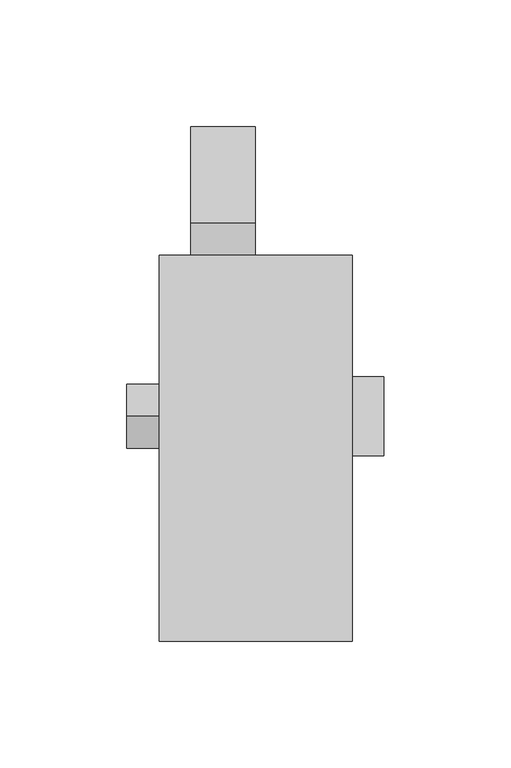
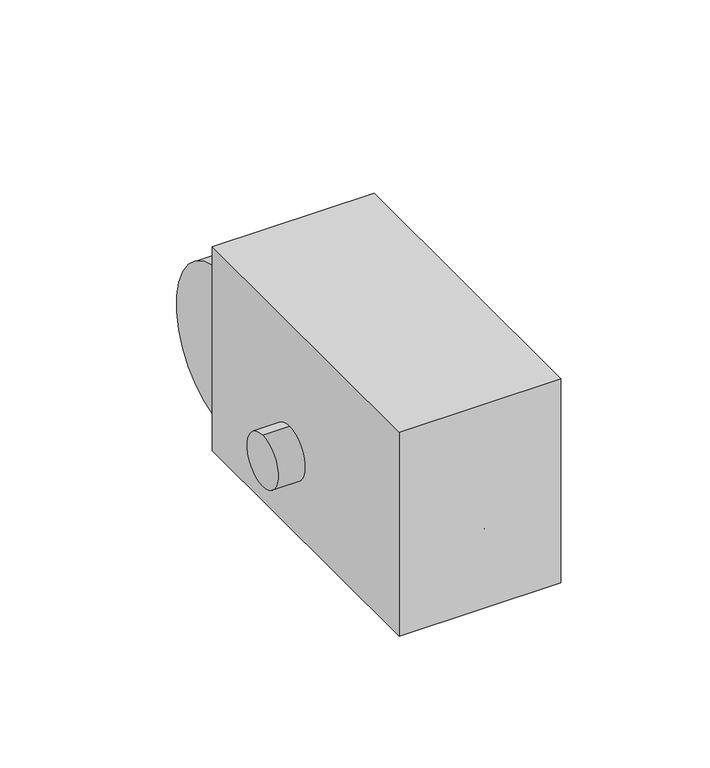
"""IFC4 building model written with IfcOpenShell, lengths in millimetres: proxy geometry, M0765 - Regulator, Vacuum : M0765 - Regulator, Vacuum."""

import ifcopenshell
import ifcopenshell.guid

model = None  # the IFC model being written
_history = None  # IfcOwnerHistory: only IFC2X3 demands one
_inside = {}  # id of a spatial element -> (the spatial element, [elements in it])
_under = {}  # id of a project, library or spatial element -> (it, [spatial elements below it])
_declared = {}  # id of a project -> (the project, [libraries it declares])
_typed = {}  # id of a type object -> (the type object, [elements of that type])
_made_of = {}  # id of a material, layer set ... -> (it, [elements and type objects made of it])


def new_model(schema):
    """Start an empty IFC model of exactly this schema.

    Asked for "IFC4X3", IfcOpenShell would pick the latest addendum, in which some entities
    have other attributes; the version numbers below select the first issue.
    IFC2X3 requires an IfcOwnerHistory on every rooted entity: one is made here for all.
    """
    global model, _history
    if schema == "IFC4X3":
        model = ifcopenshell.file(schema_version=(4, 3, 0, 0))
    else:
        model = ifcopenshell.file(schema=schema)
    _inside.clear()
    _under.clear()
    _declared.clear()
    _typed.clear()
    _made_of.clear()
    _history = None
    if model.schema == "IFC2X3":
        org = make("IfcOrganization", Name="unknown")
        user = make(
            "IfcPersonAndOrganization",
            ThePerson=make("IfcPerson", FamilyName="unknown"),
            TheOrganization=org,
        )
        app = make(
            "IfcApplication",
            ApplicationDeveloper=org,
            Version="unknown",
            ApplicationFullName="unknown",
            ApplicationIdentifier="unknown",
        )
        _history = make(
            "IfcOwnerHistory",
            OwningUser=user,
            OwningApplication=app,
            ChangeAction="ADDED",
            CreationDate=0,
        )
    return model


def make(cls, **values):
    """One entity of the class cls with the attributes given. An attribute that is None is left unset."""
    return model.create_entity(
        cls, **{name: value for name, value in values.items() if value is not None}
    )


def rooted(cls, **values):
    """An entity with a GlobalId (a new one), such as an element, a storey or a relation."""
    return make(cls, GlobalId=ifcopenshell.guid.new(), OwnerHistory=_history, **values)


def si_unit(unit_type, name, prefix=None):
    """IfcSIUnit, for example si_unit("LENGTHUNIT", "METRE", prefix="MILLI")."""
    return make("IfcSIUnit", UnitType=unit_type, Prefix=prefix, Name=name)


def assignment(units):
    """IfcUnitAssignment: the units of a project."""
    return None if units is None else make("IfcUnitAssignment", Units=units)


def point(xyz):
    """IfcCartesianPoint."""
    return None if xyz is None else make("IfcCartesianPoint", Coordinates=xyz)


def direction(xyz):
    """IfcDirection."""
    return None if xyz is None else make("IfcDirection", DirectionRatios=xyz)


def frame(location, z_axis=None, x_axis=None):
    """IfcAxis2Placement3D, a coordinate frame: its origin and axes. An axis left out is left unset."""
    return make(
        "IfcAxis2Placement3D",
        Location=point(location),
        Axis=direction(z_axis),
        RefDirection=direction(x_axis),
    )


def frame_2d(location, x_axis=None):
    """IfcAxis2Placement2D, a coordinate frame in the plane: its origin and x axis."""
    return make(
        "IfcAxis2Placement2D", Location=point(location), RefDirection=direction(x_axis)
    )


def origin():
    """The frame at (0, 0, 0) with its axes left unset."""
    return frame((0.0, 0.0, 0.0))


def origin_with_axes():
    """The frame at (0, 0, 0) with the z axis (0, 0, 1) and the x axis (1, 0, 0) written out."""
    return frame((0.0, 0.0, 0.0), z_axis=(0.0, 0.0, 1.0), x_axis=(1.0, 0.0, 0.0))


def place(relative_to, where):
    """IfcLocalPlacement: puts the frame where relative to a parent placement (None: the world)."""
    return make(
        "IfcLocalPlacement", PlacementRelTo=relative_to, RelativePlacement=where
    )


def context(
    kind, dimensions, precision=None, world=None, true_north=None, identifier=None
):
    """IfcGeometricRepresentationContext, for example the 3D "Model" context."""
    return make(
        "IfcGeometricRepresentationContext",
        ContextIdentifier=identifier,
        ContextType=kind,
        CoordinateSpaceDimension=dimensions,
        Precision=precision,
        WorldCoordinateSystem=world,
        TrueNorth=true_north,
    )


def project(units=None, contexts=None):
    """IfcProject with its units and contexts."""
    return rooted(
        "IfcProject",
        Name="project",
        RepresentationContexts=contexts,
        UnitsInContext=assignment(units),
    )


def spatial(cls, under=None, at=None, **own):
    """A site, building, storey or space (cls), placed at a placement, below another one or the project."""
    s = rooted(cls, ObjectPlacement=at, **own)
    if under is not None:
        _under.setdefault(under.id(), (under, []))[1].append(s)
    return s


def polyline(points):
    """IfcPolyline through the points."""
    return make("IfcPolyline", Points=[point(p) for p in points])


def circle_curve(where, radius):
    """IfcCircle in the frame where."""
    return make("IfcCircle", Position=where, Radius=radius)


def trimmed(basis, trim1, trim2, sense, master):
    """IfcTrimmedCurve: the piece of a basis curve between two trims."""
    return make(
        "IfcTrimmedCurve",
        BasisCurve=basis,
        Trim1=trim1,
        Trim2=trim2,
        SenseAgreement=sense,
        MasterRepresentation=master,
    )


def segment(curve, same_sense, transition):
    """IfcCompositeCurveSegment."""
    return make(
        "IfcCompositeCurveSegment",
        Transition=transition,
        SameSense=same_sense,
        ParentCurve=curve,
    )


def composite_curve(segments, self_intersect=None):
    """IfcCompositeCurve: segments joined end to end."""
    return make("IfcCompositeCurve", Segments=segments, SelfIntersect=self_intersect)


def outline(outer, holes=None, kind="AREA"):
    """IfcArbitraryClosedProfileDef: a profile drawn as a closed curve; with holes, ...WithVoids."""
    if holes is None:
        return make("IfcArbitraryClosedProfileDef", ProfileType=kind, OuterCurve=outer)
    return make(
        "IfcArbitraryProfileDefWithVoids",
        ProfileType=kind,
        OuterCurve=outer,
        InnerCurves=holes,
    )


def extrude(swept, where, along, depth):
    """IfcExtrudedAreaSolid: the profile swept, set in the frame where, extruded along a direction by depth."""
    return make(
        "IfcExtrudedAreaSolid",
        SweptArea=swept,
        Position=where,
        ExtrudedDirection=direction(along),
        Depth=depth,
    )


def shape(context_of_items, identifier, shape_type, items):
    """IfcShapeRepresentation: the items that make up one representation, for example the "Body"."""
    return make(
        "IfcShapeRepresentation",
        ContextOfItems=context_of_items,
        RepresentationIdentifier=identifier,
        RepresentationType=shape_type,
        Items=items,
    )


def source(mapping_origin, context_of_items, identifier, shape_type, items):
    """IfcRepresentationMap: a shape defined once, which mapped items show again and again."""
    return make(
        "IfcRepresentationMap",
        MappingOrigin=mapping_origin,
        MappedRepresentation=shape(context_of_items, identifier, shape_type, items),
    )


def transform(
    local_origin,
    x_axis=None,
    y_axis=None,
    z_axis=None,
    scale=None,
    scale2=None,
    scale3=None,
    uniform=True,
):
    """IfcCartesianTransformationOperator3D, or its non-uniform kind. x_axis, y_axis, z_axis: its Axis1, 2, 3."""
    if uniform:
        return make(
            "IfcCartesianTransformationOperator3D",
            Axis1=direction(x_axis),
            Axis2=direction(y_axis),
            LocalOrigin=point(local_origin),
            Scale=scale,
            Axis3=direction(z_axis),
        )
    return make(
        "IfcCartesianTransformationOperator3DnonUniform",
        Axis1=direction(x_axis),
        Axis2=direction(y_axis),
        LocalOrigin=point(local_origin),
        Scale=scale,
        Axis3=direction(z_axis),
        Scale2=scale2,
        Scale3=scale3,
    )


def mapped(mapping_source, mapping_target):
    """IfcMappedItem: shows the shape of a source again, moved by a transform."""
    return make(
        "IfcMappedItem", MappingSource=mapping_source, MappingTarget=mapping_target
    )


def made_of(thing, what):
    """Note that an element or type object is made of a material, layer set ...; save() writes the relation."""
    if what is not None:
        _made_of.setdefault(what.id(), (what, []))[1].append(thing)
    return thing


def element(
    cls,
    number,
    at=None,
    inside=None,
    cuts=None,
    type_object=None,
    material=None,
    context=None,
    identifier="Body",
    shape_type=None,
    held_by="IfcProductDefinitionShape",
    body=None,
    shapes=None,
    **own,
):
    """One element of the class cls, such as IfcWall. Its Tag is "e" and its number.

    at: its placement. inside: the storey or other place that contains it. cuts: it is an
    opening in that element (IfcRelVoidsElement). A single representation is given by context,
    identifier, shape_type and body (its items); several are given by shapes. held_by: the class
    of the entity that holds the representations. save() writes the other relations.
    """
    e = rooted(cls, Tag="e%d" % number, ObjectPlacement=at, **own)
    if body is not None:
        shapes = [shape(context, identifier, shape_type, body)]
    if shapes is not None:
        e.Representation = make(held_by, Representations=shapes)
    if inside is not None:
        _inside.setdefault(inside.id(), (inside, []))[1].append(e)
    if cuts is not None:
        rooted(
            "IfcRelVoidsElement", RelatingBuildingElement=cuts, RelatedOpeningElement=e
        )
    if type_object is not None:
        _typed.setdefault(type_object.id(), (type_object, []))[1].append(e)
    return made_of(e, material)


def aggregate(whole, parts):
    """IfcRelAggregates: a whole, such as a stair, and the parts it consists of."""
    return rooted("IfcRelAggregates", RelatingObject=whole, RelatedObjects=parts)


def save(model, path):
    """Write the relations noted so far, then the file.

    IfcRelAggregates (storeys below a building ...), IfcRelContainedInSpatialStructure (elements
    in a storey), IfcRelDefinesByType, IfcRelAssociatesMaterial and IfcRelDeclares: one each for
    every whole, place, type object, material and project.
    """
    for whole, parts in _under.values():
        aggregate(whole, parts)
    for where, things in _inside.values():
        rooted(
            "IfcRelContainedInSpatialStructure",
            RelatedElements=things,
            RelatingStructure=where,
        )
    for kind, things in _typed.values():
        rooted("IfcRelDefinesByType", RelatedObjects=things, RelatingType=kind)
    for what, things in _made_of.values():
        rooted("IfcRelAssociatesMaterial", RelatedObjects=things, RelatingMaterial=what)
    for by, libraries in _declared.values():
        rooted("IfcRelDeclares", RelatingContext=by, RelatedDefinitions=libraries)
    model.write(path)


def plane_surface(at):
    """IfcPlane: the flat surface through the origin of the frame at, square to its z axis."""
    return make("IfcPlane", Position=at)


def cylinder_surface(at, radius):
    """IfcCylindricalSurface: all points at the distance radius from the z axis of the frame at."""
    return make("IfcCylindricalSurface", Position=at, Radius=radius)


def revolved_surface(curve, axis_point, axis_direction):
    """IfcSurfaceOfRevolution: the curve turned about the line through axis_point along axis_direction."""
    return make(
        "IfcSurfaceOfRevolution",
        SweptCurve=make("IfcArbitraryOpenProfileDef", ProfileType="CURVE", Curve=curve),
        AxisPosition=make("IfcAxis1Placement", Location=point(axis_point), Axis=direction(axis_direction)),
    )


def advanced_brep(points, edges, surfaces, faces):
    """IfcAdvancedBrep: a solid bounded by faces that lie on surfaces and meet in shared edges.

    An edge is (start, end): straight between two places in points (the first is 0);
    or (start, end, curve); or (start, end, curve, False) where it runs against its curve.
    A face is (place in surfaces, loops), or (place, loops, False) where it looks against
    its surface's normal. A loop lists edges by number (the first is 1), with a minus sign
    where the edge is run from its end to its start. The first loop is the outer one.
    """
    corners = [point(p) for p in points]
    vertices = [make("IfcVertexPoint", VertexGeometry=c) for c in corners]
    made = []
    for start, end, *more in edges:
        made.append(
            make(
                "IfcEdgeCurve",
                EdgeStart=vertices[start],
                EdgeEnd=vertices[end],
                EdgeGeometry=more[0] if more else make("IfcPolyline", Points=[corners[start], corners[end]]),
                SameSense=more[1] if len(more) > 1 else True,
            )
        )
    hull = []
    for where, loops, *sense in faces:
        bounds = []
        for j, loop in enumerate(loops):
            ring = [make("IfcOrientedEdge", EdgeElement=made[abs(k) - 1], Orientation=k > 0) for k in loop]
            bounds.append(
                make(
                    "IfcFaceOuterBound" if j == 0 else "IfcFaceBound",
                    Bound=make("IfcEdgeLoop", EdgeList=ring),
                    Orientation=True,
                )
            )
        hull.append(make("IfcAdvancedFace", Bounds=bounds, FaceSurface=surfaces[where], SameSense=sense[0] if sense else True))
    return make("IfcAdvancedBrep", Outer=make("IfcClosedShell", CfsFaces=hull))


def specialty_equipment_494a7e5c(model_context):
    return source(origin(), model_context, "Body", "SolidModel", [
        extrude(outline(polyline([(38.1, 152.4), (38.1, 0.0), (-38.1, 0.0), (-38.1, 152.4), (38.1, 152.4)])), origin_with_axes(), (0.0, 0.0, 1.0), 101.6),
        advanced_brep(
        [(-0.2368425, 76.2, 53.3223414), (-0.2368425, 76.2, 22.8776586), (-0.2368425, 76.2, 38.1), (-0.2368425, 31.8738169, 53.3223414), (-0.2368425, 31.8738169, 22.8776586), (-0.2368425, 31.8738169, 43.8248613), (-0.2368425, 31.8738169, 32.3751387), (-0.2368425, 9.172523, 43.8248613), (-0.2368425, 9.172523, 32.3751387), (-0.2368425, 9.172523, 40.8134652), (-0.2368425, 9.172523, 35.3865348), (-0.2368425, 0.0, 40.8134652), (-0.2368425, 0.0, 35.3865348), (-0.2368425, 0.0, 38.1)],
        [
            (0, 1, circle_curve(frame((-0.2368425, 76.2, 38.1), z_axis=(0.0, 1.0, 0.0), x_axis=(0.0, 0.0, -1.0)), 15.2223414)),
            (1, 2),
            (2, 0),
            (1, 0, circle_curve(frame((-0.2368425, 76.2, 38.1), z_axis=(0.0, 1.0, 0.0), x_axis=(0.0, 0.0, -1.0)), 15.2223414)),
            (3, 4, circle_curve(frame((-0.2368425, 31.8738169, 38.1), z_axis=(0.0, 1.0, 0.0), x_axis=(0.0, 0.0, -1.0)), 15.2223414)),
            (4, 1),
            (0, 3),
            (4, 3, circle_curve(frame((-0.2368425, 31.8738169, 38.1), z_axis=(0.0, 1.0, 0.0), x_axis=(0.0, 0.0, -1.0)), 15.2223414)),
            (5, 6, circle_curve(frame((-0.2368425, 31.8738169, 38.1), z_axis=(0.0, 1.0, 0.0), x_axis=(0.0, 0.0, -1.0)), 5.7248613)),
            (6, 4),
            (3, 5),
            (6, 5, circle_curve(frame((-0.2368425, 31.8738169, 38.1), z_axis=(0.0, 1.0, 0.0), x_axis=(0.0, 0.0, -1.0)), 5.7248613)),
            (7, 8, circle_curve(frame((-0.2368425, 9.172523, 38.1), z_axis=(0.0, 1.0, 0.0), x_axis=(0.0, 0.0, -1.0)), 5.7248613)),
            (8, 6),
            (5, 7),
            (8, 7, circle_curve(frame((-0.2368425, 9.172523, 38.1), z_axis=(0.0, 1.0, 0.0), x_axis=(0.0, 0.0, -1.0)), 5.7248613)),
            (9, 10, circle_curve(frame((-0.2368425, 9.172523, 38.1), z_axis=(0.0, 1.0, 0.0), x_axis=(0.0, 0.0, -1.0)), 2.7134652)),
            (10, 8),
            (7, 9),
            (10, 9, circle_curve(frame((-0.2368425, 9.172523, 38.1), z_axis=(0.0, 1.0, 0.0), x_axis=(0.0, 0.0, -1.0)), 2.7134652)),
            (11, 12, circle_curve(frame((-0.2368425, 0.0, 38.1), z_axis=(0.0, 1.0, 0.0), x_axis=(0.0, 0.0, -1.0)), 2.7134652)),
            (12, 10),
            (9, 11),
            (12, 11, circle_curve(frame((-0.2368425, 0.0, 38.1), z_axis=(0.0, 1.0, 0.0), x_axis=(0.0, 0.0, -1.0)), 2.7134652)),
            (13, 12),
            (11, 13),
        ],
        [
            plane_surface(frame((-0.2368425, 76.2, 38.1), z_axis=(0.0, 1.0, 0.0), x_axis=(0.0, 0.0, -1.0))),
            cylinder_surface(frame((-0.2368425, 1297.7300755, 38.1), z_axis=(0.0, -1.0, 0.0), x_axis=(0.0, 0.0, -1.0)), 15.2223414),
            plane_surface(frame((-0.2368425, 31.8738169, 38.1), z_axis=(0.0, -1.0, 0.0), x_axis=(0.0, 0.0, -1.0))),
            cylinder_surface(frame((-0.2368425, 1297.7300755, 38.1), z_axis=(0.0, -1.0, 0.0), x_axis=(0.0, 0.0, -1.0)), 5.7248613),
            plane_surface(frame((-0.2368425, 9.172523, 38.1), z_axis=(0.0, -1.0, 0.0), x_axis=(0.0, 0.0, -1.0))),
            cylinder_surface(frame((-0.2368425, 1297.7300755, 38.1), z_axis=(0.0, -1.0, 0.0), x_axis=(0.0, 0.0, -1.0)), 2.7134652),
            plane_surface(frame((-0.2368425, 0.0, 38.1), z_axis=(0.0, -1.0, 0.0), x_axis=(0.0, 0.0, -1.0))),
        ],
        [
            (0, [[1, 2, 3]]),
            (0, [[4, -3, -2]]),
            (1, [[5, 6, -1, 7]]),
            (1, [[8, -7, -4, -6]]),
            (2, [[9, 10, -5, 11]]),
            (2, [[12, -11, -8, -10]]),
            (3, [[13, 14, -9, 15]]),
            (3, [[16, -15, -12, -14]]),
            (4, [[17, 18, -13, 19]]),
            (4, [[20, -19, -16, -18]]),
            (5, [[21, 22, -17, 23]]),
            (5, [[24, -23, -20, -22]]),
            (6, [[25, -21, 26]]),
            (6, [[-26, -24, -25]]),
        ],
    ),
        advanced_brep(
        [(50.5631575, 104.5493597, 38.1), (50.5631575, 73.2506403, 38.1), (22.2137978, 73.2506403, 38.1), (22.2137978, 104.5493597, 38.1), (50.5631575, 88.9, 38.1), (-0.2368425, 127.0, 38.1), (-0.2368425, 50.8, 38.1), (-0.2368425, 88.9, 38.1)],
        [
            (0, 1, circle_curve(frame((50.5631575, 88.9, 38.1), z_axis=(-1.0, 0.0, 0.0), x_axis=(0.0, -1.0, 0.0)), 15.6493597)),
            (1, 2),
            (2, 3, circle_curve(frame((22.2137978, 88.9, 38.1), z_axis=(1.0, 0.0, 0.0), x_axis=(0.0, -1.0, 0.0)), 15.6493597)),
            (3, 0),
            (1, 0, circle_curve(frame((50.5631575, 88.9, 38.1), z_axis=(-1.0, 0.0, 0.0), x_axis=(0.0, -1.0, 0.0)), 15.6493597)),
            (3, 2, circle_curve(frame((22.2137978, 88.9, 38.1), z_axis=(1.0, 0.0, 0.0), x_axis=(0.0, -1.0, 0.0)), 15.6493597)),
            (4, 1),
            (0, 4),
            (5, 6, circle_curve(frame((-0.2368425, 88.9, 38.1), z_axis=(-1.0, 0.0, 0.0), x_axis=(0.0, -1.0, 0.0)), 38.1)),
            (6, 7),
            (7, 5),
            (6, 5, circle_curve(frame((-0.2368425, 88.9, 38.1), z_axis=(-1.0, 0.0, 0.0), x_axis=(0.0, -1.0, 0.0)), 38.1)),
            (2, 6),
            (5, 3),
        ],
        [
            cylinder_surface(frame((-51.0368425, 88.9, 38.1), z_axis=(1.0, 0.0, 0.0), x_axis=(0.0, -1.0, 0.0)), 15.6493597),
            plane_surface(frame((50.5631575, 88.9, 38.1), z_axis=(1.0, 0.0, 0.0), x_axis=(0.0, -1.0, 0.0))),
            plane_surface(frame((-0.2368425, 88.9, 38.1), z_axis=(-1.0, 0.0, 0.0), x_axis=(0.0, -1.0, 0.0))),
            revolved_surface(polyline([(-0.2368425, 50.8, 38.1), (22.2137978, 73.2506403, 38.1)]), (-51.0368425, 88.9, 38.1), (1.0, 0.0, 0.0)),
        ],
        [
            (0, [[1, 2, 3, 4]]),
            (0, [[5, -4, 6, -2]]),
            (1, [[7, -1, 8]]),
            (1, [[-8, -5, -7]]),
            (2, [[9, 10, 11]]),
            (2, [[12, -11, -10]]),
            (3, [[-3, 13, -9, 14]]),
            (3, [[-6, -14, -12, -13]]),
        ],
    ),
        extrude(outline(composite_curve([segment(trimmed(circle_curve(frame_2d((88.9, 38.1)), 12.7), [point((88.9, 25.4))], [point((88.9, 50.8))], False, "CARTESIAN"), True, "CONTINUOUS"), segment(trimmed(circle_curve(frame_2d((88.9, 38.1)), 12.7), [point((88.9, 50.8))], [point((88.9, 25.4))], False, "CARTESIAN"), True, "CONTINUOUS")], self_intersect=False)), frame((-51.0368425, 0.0, 0.0), z_axis=(1.0, 0.0, 0.0), x_axis=(0.0, 1.0, 0.0)), (0.0, 0.0, 1.0), 50.8),
        extrude(outline(composite_curve([segment(trimmed(circle_curve(frame_2d((69.85, 19.05)), 19.05), [point((69.85, 0.0))], [point((50.8, 19.05))], False, "CARTESIAN"), True, "CONTINUOUS"), segment(polyline([(50.8, 19.05), (50.8, 57.15)]), True, "CONTINUOUS"), segment(trimmed(circle_curve(frame_2d((69.85, 57.15)), 19.05), [point((50.8, 57.15))], [point((69.85, 76.2))], False, "CARTESIAN"), True, "CONTINUOUS"), segment(polyline([(69.85, 76.2), (107.95, 76.2)]), True, "CONTINUOUS"), segment(trimmed(circle_curve(frame_2d((107.95, 57.15)), 19.05), [point((107.95, 76.2))], [point((127.0, 57.15))], False, "CARTESIAN"), True, "CONTINUOUS"), segment(polyline([(127.0, 57.15), (127.0, 19.05)]), True, "CONTINUOUS"), segment(trimmed(circle_curve(frame_2d((107.95, 19.05)), 19.05), [point((127.0, 19.05))], [point((107.95, 0.0))], False, "CARTESIAN"), True, "CONTINUOUS"), segment(polyline([(107.95, 0.0), (69.85, 0.0)]), True, "CONTINUOUS")], self_intersect=False)), frame((-25.6368425, 0.0, 0.0), z_axis=(1.0, 0.0, 0.0), x_axis=(0.0, 1.0, 0.0)), (0.0, 0.0, 1.0), 25.4),
        extrude(outline(composite_curve([segment(trimmed(circle_curve(frame_2d((165.1, 38.1)), 38.1), [point((165.1, 0.0))], [point((165.1, 76.2))], False, "CARTESIAN"), True, "CONTINUOUS"), segment(trimmed(circle_curve(frame_2d((165.1, 38.1)), 38.1), [point((165.1, 76.2))], [point((165.1, 0.0))], False, "CARTESIAN"), True, "CONTINUOUS")], self_intersect=False)), frame((-25.6368425, 0.0, 0.0), z_axis=(1.0, 0.0, 0.0), x_axis=(0.0, 1.0, 0.0)), (0.0, 0.0, 1.0), 25.4),
    ])


if __name__ == "__main__":
    model = new_model("IFC4")
    model_context = context("Model", 3, world=origin())
    ifc_project = project(units=[si_unit("LENGTHUNIT", "METRE", prefix="MILLI")], contexts=[model_context])
    site = spatial("IfcSite", under=ifc_project)
    building = spatial("IfcBuilding", under=site)
    placement = place(None, origin())
    specialty_equipment_shape = specialty_equipment_494a7e5c(model_context)
    element("IfcBuildingElementProxy", 1, Name="M0765 - Regulator, Vacuum : M0765 - Regulator, Vacuum", ObjectType="M0765 - Regulator, Vacuum : M0765 - Regulator, Vacuum", at=placement, inside=building, context=model_context, shape_type="MappedRepresentation", body=[
        mapped(specialty_equipment_shape, transform((0.0, 0.0, 0.0), x_axis=(1.0, 0.0, 0.0), y_axis=(0.0, 1.0, 0.0), z_axis=(0.0, 0.0, 1.0))),
    ])
    save(model, "model.ifc")

# Revit data of these elements
# Type "M0765 - Regulator, Vacuum : M0765 - Regulator, Vacuum"
#   Watts2 = "0"
#   Watts1 = "0"
#   Unit_Issue = "EA"
#   UTIL_6_Misc = "-"
#   UTIL_5_NonMedGas = "-"
#   UTIL_4_MiscGas = "-"
#   UTIL_3_MedGas = "B"
#   UTIL_2_Elec = "-"
#   UTIL_1_WaterDrain = "-"
#   Nomenclature = "Regulator, Vacuum"
#   NSN = "6515"
#   Location [instance default] = ""
#   JSN = "M0765"
#   Fund_Source_VA = "-"
#   Fund_Source_Navy = "-"
#   Fund_Source_Army = "-"
#   Fund_Source_AF = "-"
#   ELEC_Volts2 = "0"
#   ELEC_Volts1 = "0"
#   ELEC_Phase2 = "0"
#   ELEC_Phase1 = "0"
#   ELEC_HertzSwitch = "0"
#   ELEC_HertzDependent = "0"
#   ELEC_Hertz = "0"
#   ELEC_Amps2 = "0"
#   ELEC_Amps1 = "0"
#   DetailDescription = "Vacuum pressure regulator for connection to central piped vacuum system. Standard display scale is graduated at least from 0 to 200 mm Hg of vacuum. Displays on specialized regulators may cover other vacuum ranges. Regulator type (continuous, intermittent, continuous/intermittent, surgical, pediatric, thoracic, etc.) as required. To be used in delivery, neonatal, pediatrics or any area where suction is required. Database pricing reflects continuous regulators graduated to 200 mm Hg with a full line vacuum selection switch and DISS configured inlets and outlets."
#   CAT_VA = "C"
#   CAT_Navy = "C"
#   CAT_IHS = "-"
#   CAT_Army = "C"
#   CAT_AF = "C"
#   BTUperhour = "0"
#   Weight_IP = 1
#   Default Elevation = 4' - 0"
#   DIM_Width_IP = 0' - 3"
#   DIM_Height_IP = 0' - 6"
#   DIM_Depth_IP = 0' - 4"
#   finish [instance default] = none
# Element 1 (IfcBuildingElementProxy, "M0765 - Regulator, Vacuum : M0765 - Regulator, Vacuum")
#   Location = "ORGS1"
#   Materials on its faces: "EquipSpace"
# Materials
#   "EquipSpace": class "Unassigned", colour RGB 221 217 195, transparency 0.5
